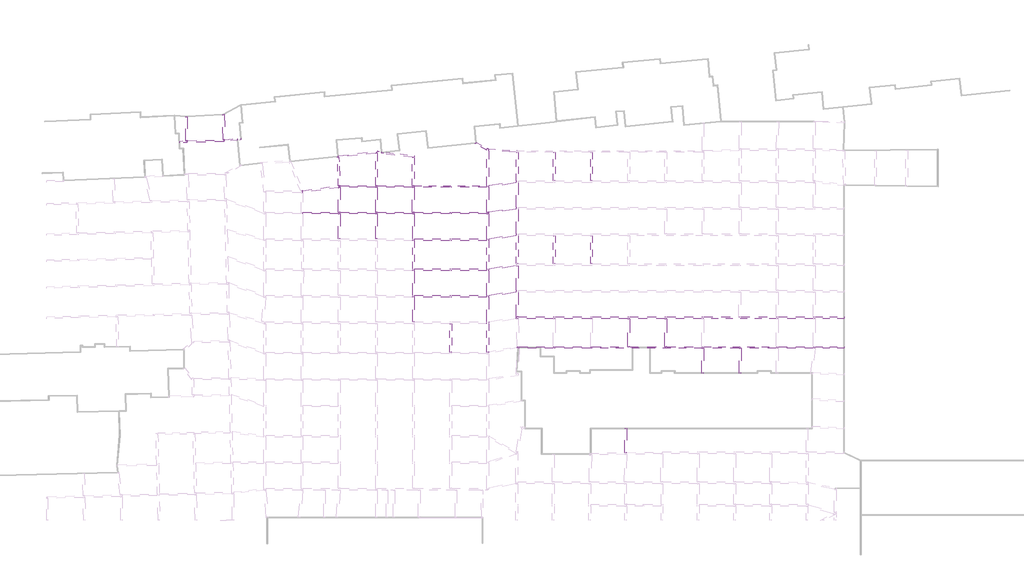
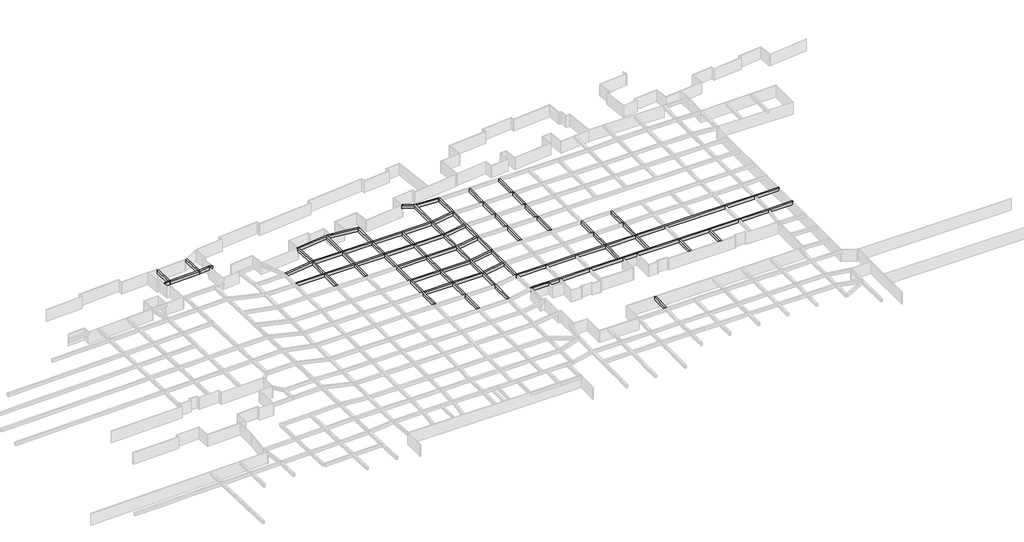
# One storey, part 19 of 20: 47 beams.
"""IFC4 building model written with IfcOpenShell, lengths in millimetres."""

from ifc_helpers import new_model, si_unit, frame, origin, place, context, project, spatial, polyline, outline, extrude, faceted_brep, element, save

model = new_model("IFC4")

# Units and contexts
model_context = context("Model", 3, world=origin())
ifc_project = project(units=[si_unit("LENGTHUNIT", "METRE", prefix="MILLI")], contexts=[model_context])

# Site, building, storey
site = spatial("IfcSite", under=ifc_project)
building = spatial("IfcBuilding", under=site)
storey = spatial("IfcBuildingStorey", under=building, Name="户型图", Elevation=0.0)

# Beams
placement = place(None, origin())
element("IfcBeam", 1, ObjectType="混凝土 - 矩形梁 : KL_beam", at=placement, inside=storey, context=model_context, shape_type="Brep", body=[
    faceted_brep([(37889.2589786, 194514.8382206, 3300.0), (37874.207263, 194914.598332, 3300.0), (37644.5215781, 194902.5610153, 3300.0), (36273.4586739, 194830.7066533, 3300.0), (36294.3930564, 194431.2548394, 3300.0), (37889.2589786, 194514.8382206, 2500.0), (36294.3930564, 194431.2548394, 2500.0), (37874.207263, 194914.598332, 2500.0), (36273.4586739, 194830.7066533, 2500.0), (37644.5215781, 194902.5610153, 2500.0)], [[[0, 1, 2, 3, 4]], [[5, 0, 4, 6]], [[7, 5, 6, 8, 9]], [[1, 7, 9, 8, 3, 2]], [[4, 3, 8, 6]], [[1, 0, 5, 7]]]),
])
element("IfcBeam", 2, ObjectType="混凝土 - 矩形梁 : KL_beam", at=placement, inside=storey, context=model_context, shape_type="Brep", body=[
    faceted_brep([(45868.2351761, 195097.7600189, 3300.0), (45638.7989465, 195092.5031037, 3300.0), (38044.2614823, 194918.4946679, 3300.0), (37874.207263, 194914.598332, 3300.0), (37889.2589786, 194514.8382206, 3300.0), (45893.7648239, 194698.2399811, 3300.0), (37889.2589786, 194514.8382206, 2500.0), (45893.7648239, 194698.2399811, 2500.0), (37874.207263, 194914.598332, 2500.0), (38044.2614823, 194918.4946679, 2500.0), (45638.7989465, 195092.5031037, 2500.0), (45868.2351761, 195097.7600189, 2500.0)], [[[0, 1, 2, 3, 4, 5]], [[5, 4, 6, 7]], [[7, 6, 8, 9, 10, 11]], [[3, 2, 1, 0, 11, 10, 9, 8]], [[3, 8, 6, 4]], [[0, 5, 7, 11]]]),
])
element("IfcBeam", 3, ObjectType="混凝土 - 矩形梁 : KL_beam", at=placement, inside=storey, context=model_context, shape_type="Brep", body=[
    faceted_brep([(45868.2351761, 195097.7600189, 3300.0), (45893.7648239, 194698.2399811, 3300.0), (48684.0697224, 194991.5128437, 3300.0), (48667.2783502, 195165.2272583, 3300.0), (48786.7216498, 195176.7727417, 3300.0), (48803.4165187, 195004.0566974, 3300.0), (49600.2651229, 195087.8088606, 3300.0), (49582.7742245, 195254.2236424, 3300.0), (49463.4315971, 195241.6802268, 3300.0), (49439.1111102, 195473.0742031, 3300.0), (46038.3737549, 195115.6423041, 3300.0), (49600.2651229, 195087.8088606, 2500.0), (48803.4165187, 195004.0566974, 2500.0), (45893.7648239, 194698.2399811, 2500.0), (45868.2351761, 195097.7600189, 2500.0), (46038.3737549, 195115.6423041, 2500.0), (49439.1111102, 195473.0742031, 2500.0), (49463.4315971, 195241.6802268, 2500.0), (49582.7742245, 195254.2236424, 2500.0), (48786.7216498, 195176.7727417, 2500.0), (48667.2783502, 195165.2272583, 2500.0), (48684.0697224, 194991.5128437, 2500.0)], [[[0, 1, 2, 3, 4, 5, 6, 7, 8, 9, 10]], [[11, 6, 5, 12]], [[13, 14, 15, 16, 17, 18, 11, 12, 19, 20, 21]], [[14, 0, 10, 9, 16, 15]], [[6, 11, 18, 7]], [[0, 14, 13, 1]], [[8, 17, 16, 9]], [[17, 8, 7, 18]], [[20, 3, 2, 21]], [[4, 19, 12, 5]], [[3, 20, 19, 4]], [[1, 13, 21, 2]]]),
])
element("IfcBeam", 4, ObjectType="混凝土 - 矩形梁 : KL_beam", at=placement, inside=storey, context=model_context, shape_type="SweptSolid", body=[
    extrude(outline(polyline([(37724.3604177, 200089.1615243), (37925.547951, 200099.7053161), (38044.2614823, 194918.4946679), (37874.207263, 194914.598332), (37644.5215781, 194902.5610153), (37525.4456991, 200099.586203), (37724.3604177, 200089.1615243)])), frame((0.0, 0.0, 2500.0), z_axis=(0.0, 0.0, 1.0), x_axis=(1.0, 0.0, 0.0)), (0.0, 0.0, 1.0), 800.0),
])
element("IfcBeam", 5, ObjectType="混凝土 - 矩形梁 : KL_beam", at=placement, inside=storey, context=model_context, shape_type="SweptSolid", body=[
    extrude(outline(polyline([(45729.8203033, 200508.709899), (45912.5795901, 200605.8847355), (46038.3737549, 195115.6423041), (45868.2351761, 195097.7600189), (45638.7989465, 195092.5031037), (45514.9591113, 200497.4495011), (45729.8203033, 200508.709899)])), frame((0.0, 0.0, 2500.0), z_axis=(0.0, 0.0, 1.0), x_axis=(1.0, 0.0, 0.0)), (0.0, 0.0, 1.0), 800.0),
])
element("IfcBeam", 6, ObjectType="混凝土 - 矩形梁 : KL_beam", at=placement, inside=storey, context=model_context, shape_type="Brep", body=[
    faceted_brep([(86850.0, 179140.0, 3300.0), (86850.0, 179540.0, 3300.0), (86806.9296004, 179540.0, 3300.0), (86406.9296004, 179540.0, 3300.0), (78866.5603873, 179540.0, 3300.0), (78466.5603873, 179540.0, 3300.0), (70871.1713568, 179540.0, 3300.0), (70471.1713568, 179540.0, 3300.0), (62850.0, 179540.0, 3300.0), (62850.0, 179140.0, 3300.0), (70471.1713568, 179140.0, 3300.0), (70871.1713568, 179140.0, 3300.0), (78466.5603873, 179140.0, 3300.0), (78866.5603873, 179140.0, 3300.0), (86450.0, 179140.0, 3300.0), (86850.0, 179140.0, 2500.0), (62850.0, 179140.0, 2500.0), (70471.1713568, 179140.0, 2500.0), (70871.1713568, 179140.0, 2500.0), (78466.5603873, 179140.0, 2500.0), (78866.5603873, 179140.0, 2500.0), (86450.0, 179140.0, 2500.0), (86850.0, 179540.0, 2500.0), (62850.0, 179540.0, 2500.0), (70471.1713568, 179540.0, 2500.0), (70871.1713568, 179540.0, 2500.0), (78466.5603873, 179540.0, 2500.0), (78866.5603873, 179540.0, 2500.0), (86406.9296004, 179540.0, 2500.0), (86806.9296004, 179540.0, 2500.0)], [[[0, 1, 2, 3, 4, 5, 6, 7, 8, 9, 10, 11, 12, 13, 14]], [[15, 0, 14, 13, 12, 11, 10, 9, 16, 17, 18, 19, 20, 21]], [[22, 15, 21, 20, 19, 18, 17, 16, 23, 24, 25, 26, 27, 28, 29]], [[1, 22, 29, 28, 27, 26, 25, 24, 23, 8, 7, 6, 5, 4, 3, 2]], [[9, 8, 23, 16]], [[1, 0, 15, 22]]]),
])
element("IfcBeam", 7, ObjectType="混凝土 - 矩形梁 : KL_beam", at=placement, inside=storey, context=model_context, shape_type="Brep", body=[
    faceted_brep([(70657.1859944, 185242.3021178, 3300.0), (70464.4923556, 185215.2207929, 3300.0), (62777.6028574, 184134.8989266, 3300.0), (62636.0146376, 184115.0, 3300.0), (62850.0, 184115.0, 3300.0), (62850.0, 183741.1426524, 3300.0), (70471.1713568, 184812.2284363, 3300.0), (70685.1567192, 184842.3021178, 3300.0), (62850.0, 183741.1426524, 2500.0), (70471.1713568, 184812.2284363, 2500.0), (70685.1567192, 184842.3021178, 2500.0), (62850.0, 184115.0, 2500.0), (62636.0146376, 184115.0, 2500.0), (62777.6028574, 184134.8989266, 2500.0), (70464.4923556, 185215.2207929, 2500.0), (70657.1859944, 185242.3021178, 2500.0)], [[[0, 1, 2, 3, 4, 5, 6, 7]], [[7, 6, 5, 8, 9, 10]], [[10, 9, 8, 11, 12, 13, 14, 15]], [[3, 2, 1, 0, 15, 14, 13, 12]], [[11, 4, 3, 12]], [[4, 11, 8, 5]], [[0, 7, 10, 15]]]),
])
element("IfcBeam", 8, ObjectType="混凝土 - 矩形梁 : KL_beam", at=placement, inside=storey, context=model_context, shape_type="Brep", body=[
    faceted_brep([(70657.1859944, 185242.3021178, 3300.0), (70685.1567192, 184842.3021178, 3300.0), (70871.1713568, 184842.3021178, 3300.0), (78466.5603873, 184842.3021178, 3300.0), (78866.5603873, 184842.3021178, 3300.0), (86406.9296004, 184842.3021178, 3300.0), (86806.9296004, 184842.3021178, 3300.0), (86806.9296004, 185242.3021178, 3300.0), (86406.9296004, 185242.3021178, 3300.0), (78866.5603873, 185242.3021178, 3300.0), (78466.5603873, 185242.3021178, 3300.0), (70863.7543579, 185242.3021178, 3300.0), (70685.1567192, 184842.3021178, 2500.0), (70871.1713568, 184842.3021178, 2500.0), (78466.5603873, 184842.3021178, 2500.0), (78866.5603873, 184842.3021178, 2500.0), (86406.9296004, 184842.3021178, 2500.0), (86806.9296004, 184842.3021178, 2500.0), (70657.1859944, 185242.3021178, 2500.0), (70863.7543579, 185242.3021178, 2500.0), (78466.5603873, 185242.3021178, 2500.0), (78866.5603873, 185242.3021178, 2500.0), (86406.9296004, 185242.3021178, 2500.0), (86806.9296004, 185242.3021178, 2500.0)], [[[0, 1, 2, 3, 4, 5, 6, 7, 8, 9, 10, 11]], [[1, 12, 13, 14, 15, 16, 17, 6, 5, 4, 3, 2]], [[12, 18, 19, 20, 21, 22, 23, 17, 16, 15, 14, 13]], [[18, 0, 11, 10, 9, 8, 7, 23, 22, 21, 20, 19]], [[0, 18, 12, 1]], [[7, 6, 17, 23]]]),
])
element("IfcBeam", 9, ObjectType="混凝土 - 矩形梁 : KL_beam", at=placement, inside=storey, context=model_context, shape_type="Brep", body=[
    faceted_brep([(70707.0899583, 189386.9587472, 3300.0), (70508.8980465, 191272.6288285, 3300.0), (70494.4229915, 191410.349777, 3300.0), (70231.283324, 191384.9144894, 3300.0), (70464.4923556, 185215.2207929, 3300.0), (70657.1859944, 185242.3021178, 3300.0), (70863.7543579, 185242.3021178, 3300.0), (70464.4923556, 185215.2207929, 2500.0), (70231.283324, 191384.9144894, 2500.0), (70494.4229915, 191410.349777, 2500.0), (70508.8980465, 191272.6288285, 2500.0), (70707.0899583, 189386.9587472, 2500.0), (70863.7543579, 185242.3021178, 2500.0), (70657.1859944, 185242.3021178, 2500.0)], [[[0, 1, 2, 3, 4, 5, 6]], [[7, 4, 3, 8]], [[8, 9, 10, 11, 12, 13, 7]], [[11, 0, 6, 12]], [[0, 11, 10, 9, 2, 1]], [[2, 9, 8, 3]], [[5, 4, 7, 13]], [[6, 5, 13, 12]]]),
])
element("IfcBeam", 10, ObjectType="混凝土 - 矩形梁 : KL_beam", at=placement, inside=storey, context=model_context, shape_type="Brep", body=[
    faceted_brep([(78817.8126499, 192695.8391898, 3300.0), (70467.0802921, 191670.498184, 3300.0), (70494.4229915, 191410.349777, 3300.0), (70508.8980465, 191272.6288285, 3300.0), (78466.5603873, 192249.7069048, 3300.0), (78866.5603873, 192298.8207291, 3300.0), (78822.4430306, 192658.1277652, 3300.0), (70508.8980465, 191272.6288285, 2500.0), (78466.5603873, 192249.7069048, 2500.0), (78866.5603873, 192298.8207291, 2500.0), (70467.0802921, 191670.498184, 2500.0), (78817.8126499, 192695.8391898, 2500.0), (78822.4430306, 192658.1277652, 2500.0), (70494.4229915, 191410.349777, 2500.0)], [[[0, 1, 2, 3, 4, 5, 6]], [[5, 4, 3, 7, 8, 9]], [[10, 11, 12, 9, 8, 7, 13]], [[1, 0, 11, 10]], [[1, 10, 13, 7, 3, 2]], [[0, 6, 5, 9, 12, 11]]]),
    faceted_brep([(70221.627692, 191640.3603943, 3300.0), (70221.627692, 191640.3603943, 2500.0), (70226.7428774, 191505.0349014, 2500.0), (70226.7428774, 191505.0349014, 3300.0), (70347.9566108, 191655.8716351, 2500.0), (70347.9566108, 191655.8716351, 3300.0), (70362.4316658, 191518.1506866, 3300.0), (70362.4316658, 191518.1506866, 2500.0)], [[[0, 1, 2, 3]], [[4, 5, 6, 7]], [[1, 0, 5, 4]], [[6, 3, 2, 7]], [[5, 0, 3, 6]], [[1, 4, 7, 2]]]),
])
element("IfcBeam", 11, ObjectType="混凝土 - 矩形梁 : KL_beam", at=placement, inside=storey, context=model_context, shape_type="Brep", body=[
    faceted_brep([(78866.5603873, 192298.8207291, 3300.0), (78466.5603873, 192249.7069048, 3300.0), (78466.5603873, 185242.3021178, 3300.0), (78866.5603873, 185242.3021178, 3300.0), (78866.5603873, 192249.7069048, 3300.0), (78466.5603873, 192249.7069048, 2500.0), (78466.5603873, 185242.3021178, 2500.0), (78866.5603873, 192298.8207291, 2500.0), (78866.5603873, 192249.7069048, 2500.0), (78866.5603873, 185242.3021178, 2500.0)], [[[0, 1, 2, 3, 4]], [[1, 5, 6, 2]], [[5, 7, 8, 9, 6]], [[7, 0, 4, 3, 9, 8]], [[1, 0, 7, 5]], [[3, 2, 6, 9]]]),
])
element("IfcBeam", 12, ObjectType="混凝土 - 矩形梁 : KL_beam", at=placement, inside=storey, context=model_context, shape_type="Brep", body=[
    faceted_brep([(79847.9790856, 192432.6191009, 3300.0), (80284.9846417, 192478.5502357, 3300.0), (79837.3750476, 192533.5097832, 3300.0), (80284.9846417, 192478.5502357, 2500.0), (79847.9790856, 192432.6191009, 2500.0), (79837.3750476, 192533.5097832, 2500.0)], [[[0, 1, 2]], [[3, 4, 5]], [[3, 1, 0, 4]], [[1, 3, 5, 2]], [[0, 2, 5, 4]]]),
    faceted_brep([(78866.5603873, 192249.7069048, 3300.0), (78866.5603873, 192249.7069048, 2500.0), (86406.9296004, 191323.8659819, 2500.0), (86806.9296004, 191274.7521575, 2500.0), (86806.9296004, 191274.7521575, 3300.0), (86406.9296004, 191323.8659819, 3300.0), (80814.4577688, 192413.5391103, 2500.0), (80814.4577688, 192413.5391103, 3300.0), (86806.9296004, 191677.7560877, 3300.0), (86806.9296004, 191677.7560877, 2500.0), (78866.5603873, 192298.8207291, 3300.0), (78822.4430306, 192658.1277652, 3300.0), (78822.4430306, 192658.1277652, 2500.0), (78866.5603873, 192298.8207291, 2500.0), (79741.1798737, 192300.7330579, 2500.0), (79741.1798737, 192300.7330579, 3300.0), (79715.1365445, 192548.5187841, 2500.0), (79715.1365445, 192548.5187841, 3300.0), (79728.6364581, 192420.0756853, 3300.0)], [[[0, 1, 2, 3, 4, 5]], [[6, 7, 8, 9]], [[10, 11, 12, 13]], [[0, 10, 13, 1]], [[14, 15, 7, 6]], [[15, 14, 16, 17, 18]], [[11, 10, 0, 5, 4, 8, 7, 15, 18, 17]], [[13, 12, 16, 14, 6, 9, 3, 2, 1]], [[12, 11, 17, 16]], [[8, 4, 3, 9]]]),
])
element("IfcBeam", 13, ObjectType="混凝土 - 矩形梁 : KL_beam", at=placement, inside=storey, context=model_context, shape_type="SweptSolid", body=[
    extrude(outline(polyline([(86806.9296004, 185242.3021178), (86406.9296004, 185242.3021178), (86406.9296004, 191323.8659819), (86806.9296004, 191274.7521575), (86806.9296004, 185242.3021178)])), frame((0.0, 0.0, 2500.0), z_axis=(0.0, 0.0, 1.0), x_axis=(1.0, 0.0, 0.0)), (0.0, 0.0, 1.0), 800.0),
])
element("IfcBeam", 14, ObjectType="混凝土 - 矩形梁 : KL_beam", at=placement, inside=storey, context=model_context, shape_type="Brep", body=[
    faceted_brep([(70871.1713568, 184842.3021178, 3300.0), (70685.1567192, 184842.3021178, 3300.0), (70479.6799144, 184813.4242361, 3300.0), (70471.1713568, 184812.2284363, 3300.0), (70471.1713568, 179540.0, 3300.0), (70871.1713568, 179540.0, 3300.0), (70471.1713568, 184812.2284363, 2500.0), (70471.1713568, 179540.0, 2500.0), (70685.1567192, 184842.3021178, 2500.0), (70871.1713568, 184842.3021178, 2500.0), (70871.1713568, 179540.0, 2500.0), (70479.6799144, 184813.4242361, 2500.0)], [[[0, 1, 2, 3, 4, 5]], [[3, 6, 7, 4]], [[8, 9, 10, 7, 6, 11]], [[9, 0, 5, 10]], [[6, 3, 2, 1, 8, 11]], [[1, 0, 9, 8]], [[5, 4, 7, 10]]]),
])
element("IfcBeam", 15, ObjectType="混凝土 - 矩形梁 : KL_beam", at=placement, inside=storey, context=model_context, shape_type="SweptSolid", body=[
    extrude(outline(polyline([(70871.1713568, 173790.0), (70471.1713568, 173790.0), (70471.1713568, 179140.0), (70871.1713568, 179140.0), (70871.1713568, 173790.0)])), frame((0.0, 0.0, 2500.0), z_axis=(0.0, 0.0, 1.0), x_axis=(1.0, 0.0, 0.0)), (0.0, 0.0, 1.0), 800.0),
])
element("IfcBeam", 16, ObjectType="混凝土 - 矩形梁 : KL_beam", at=placement, inside=storey, context=model_context, shape_type="SweptSolid", body=[
    extrude(outline(polyline([(78866.5603873, 179540.0), (78466.5603873, 179540.0), (78466.5603873, 184842.3021178), (78866.5603873, 184842.3021178), (78866.5603873, 179540.0)])), frame((0.0, 0.0, 2500.0), z_axis=(0.0, 0.0, 1.0), x_axis=(1.0, 0.0, 0.0)), (0.0, 0.0, 1.0), 800.0),
])
element("IfcBeam", 17, ObjectType="混凝土 - 矩形梁 : KL_beam", at=placement, inside=storey, context=model_context, shape_type="SweptSolid", body=[
    extrude(outline(polyline([(78866.5603873, 173790.0), (78466.5603873, 173790.0), (78466.5603873, 179140.0), (78866.5603873, 179140.0), (78866.5603873, 173790.0)])), frame((0.0, 0.0, 2500.0), z_axis=(0.0, 0.0, 1.0), x_axis=(1.0, 0.0, 0.0)), (0.0, 0.0, 1.0), 800.0),
])
element("IfcBeam", 18, ObjectType="混凝土 - 矩形梁 : KL_beam", at=placement, inside=storey, context=model_context, shape_type="Brep", body=[
    faceted_brep([(86450.0, 155890.0, 3300.0), (86850.0, 155890.0, 3300.0), (86850.0, 161190.0, 3300.0), (86850.0, 161590.0, 3300.0), (86850.0, 166890.0, 3300.0), (86850.0, 167290.0, 3300.0), (86850.0, 173390.0, 3300.0), (86850.0, 173790.0, 3300.0), (86850.0, 179140.0, 3300.0), (86450.0, 179140.0, 3300.0), (86450.0, 173790.0, 3300.0), (86450.0, 173390.0, 3300.0), (86450.0, 167290.0, 3300.0), (86450.0, 166890.0, 3300.0), (86450.0, 161590.0, 3300.0), (86450.0, 161190.0, 3300.0), (86450.0, 155890.0, 2500.0), (86450.0, 179140.0, 2500.0), (86450.0, 173790.0, 2500.0), (86450.0, 173390.0, 2500.0), (86450.0, 167290.0, 2500.0), (86450.0, 166890.0, 2500.0), (86450.0, 161590.0, 2500.0), (86450.0, 161190.0, 2500.0), (86850.0, 155890.0, 2500.0), (86850.0, 179140.0, 2500.0), (86850.0, 173790.0, 2500.0), (86850.0, 173390.0, 2500.0), (86850.0, 167290.0, 2500.0), (86850.0, 166890.0, 2500.0), (86850.0, 161590.0, 2500.0), (86850.0, 161190.0, 2500.0)], [[[0, 1, 2, 3, 4, 5, 6, 7, 8, 9, 10, 11, 12, 13, 14, 15]], [[16, 0, 15, 14, 13, 12, 11, 10, 9, 17, 18, 19, 20, 21, 22, 23]], [[24, 16, 23, 22, 21, 20, 19, 18, 17, 25, 26, 27, 28, 29, 30, 31]], [[1, 24, 31, 30, 29, 28, 27, 26, 25, 8, 7, 6, 5, 4, 3, 2]], [[1, 0, 16, 24]], [[9, 8, 25, 17]]]),
])
element("IfcBeam", 19, ObjectType="混凝土 - 矩形梁 : KL_beam", at=placement, inside=storey, context=model_context, shape_type="Brep", body=[
    faceted_brep([(86850.0, 161590.0, 3300.0), (86850.0, 161190.0, 3300.0), (94423.4648002, 161190.0, 3300.0), (94823.4648002, 161190.0, 3300.0), (102450.0, 161190.0, 3300.0), (102450.0, 161590.0, 3300.0), (94823.4648002, 161590.0, 3300.0), (94423.4648002, 161590.0, 3300.0), (86850.0, 161190.0, 2500.0), (94423.4648002, 161190.0, 2500.0), (94823.4648002, 161190.0, 2500.0), (102450.0, 161190.0, 2500.0), (86850.0, 161590.0, 2500.0), (94423.4648002, 161590.0, 2500.0), (94823.4648002, 161590.0, 2500.0), (102450.0, 161590.0, 2500.0)], [[[0, 1, 2, 3, 4, 5, 6, 7]], [[1, 8, 9, 10, 11, 4, 3, 2]], [[8, 12, 13, 14, 15, 11, 10, 9]], [[12, 0, 7, 6, 5, 15, 14, 13]], [[1, 0, 12, 8]], [[5, 4, 11, 15]]]),
])
element("IfcBeam", 20, ObjectType="混凝土 - 矩形梁 : KL_beam", at=placement, inside=storey, context=model_context, shape_type="Brep", body=[
    faceted_brep([(86850.0, 167290.0, 3300.0), (86850.0, 166890.0, 3300.0), (94423.4648002, 166890.0, 3300.0), (94823.4648002, 166890.0, 3300.0), (102450.0, 166890.0, 3300.0), (102450.0, 167290.0, 3300.0), (94823.4648002, 167290.0, 3300.0), (94423.4648002, 167290.0, 3300.0), (86850.0, 166890.0, 2500.0), (94423.4648002, 166890.0, 2500.0), (94823.4648002, 166890.0, 2500.0), (102450.0, 166890.0, 2500.0), (86850.0, 167290.0, 2500.0), (94423.4648002, 167290.0, 2500.0), (94823.4648002, 167290.0, 2500.0), (102450.0, 167290.0, 2500.0)], [[[0, 1, 2, 3, 4, 5, 6, 7]], [[1, 8, 9, 10, 11, 4, 3, 2]], [[8, 12, 13, 14, 15, 11, 10, 9]], [[12, 0, 7, 6, 5, 15, 14, 13]], [[1, 0, 12, 8]], [[5, 4, 11, 15]]]),
])
element("IfcBeam", 21, ObjectType="混凝土 - 矩形梁 : KL_beam", at=placement, inside=storey, context=model_context, shape_type="Brep", body=[
    faceted_brep([(86850.0, 173790.0, 3300.0), (86850.0, 173390.0, 3300.0), (94423.4648002, 173390.0, 3300.0), (94823.4648002, 173390.0, 3300.0), (102450.0, 173390.0, 3300.0), (102450.0, 173790.0, 3300.0), (94823.4648002, 173790.0, 3300.0), (94423.4648002, 173790.0, 3300.0), (86850.0, 173390.0, 2500.0), (94423.4648002, 173390.0, 2500.0), (94823.4648002, 173390.0, 2500.0), (102450.0, 173390.0, 2500.0), (86850.0, 173790.0, 2500.0), (94423.4648002, 173790.0, 2500.0), (94823.4648002, 173790.0, 2500.0), (102450.0, 173790.0, 2500.0)], [[[0, 1, 2, 3, 4, 5, 6, 7]], [[1, 8, 9, 10, 11, 4, 3, 2]], [[8, 12, 13, 14, 15, 11, 10, 9]], [[12, 0, 7, 6, 5, 15, 14, 13]], [[1, 0, 12, 8]], [[5, 4, 11, 15]]]),
])
element("IfcBeam", 22, ObjectType="混凝土 - 矩形梁 : KL_beam", at=placement, inside=storey, context=model_context, shape_type="Brep", body=[
    faceted_brep([(102850.0, 179140.0, 3300.0), (102850.0, 179170.5745823, 3300.0), (102850.0, 179540.0, 3300.0), (102450.0, 179540.0, 3300.0), (94823.4648002, 179540.0, 3300.0), (94423.4648002, 179540.0, 3300.0), (86850.0, 179540.0, 3300.0), (86850.0, 179140.0, 3300.0), (94423.4648002, 179140.0, 3300.0), (94823.4648002, 179140.0, 3300.0), (102450.0, 179140.0, 3300.0), (102850.0, 179140.0, 2500.0), (86850.0, 179140.0, 2500.0), (94423.4648002, 179140.0, 2500.0), (94823.4648002, 179140.0, 2500.0), (102450.0, 179140.0, 2500.0), (102850.0, 179540.0, 2500.0), (102850.0, 179170.5745823, 2500.0), (86850.0, 179540.0, 2500.0), (94423.4648002, 179540.0, 2500.0), (94823.4648002, 179540.0, 2500.0), (102450.0, 179540.0, 2500.0)], [[[0, 1, 2, 3, 4, 5, 6, 7, 8, 9, 10]], [[11, 0, 10, 9, 8, 7, 12, 13, 14, 15]], [[16, 17, 11, 15, 14, 13, 12, 18, 19, 20, 21]], [[2, 16, 21, 20, 19, 18, 6, 5, 4, 3]], [[7, 6, 18, 12]], [[2, 1, 0, 11, 17, 16]]]),
])
element("IfcBeam", 23, ObjectType="混凝土 - 矩形梁 : KL_beam", at=placement, inside=storey, context=model_context, shape_type="SweptSolid", body=[
    extrude(outline(polyline([(86806.9296004, 179540.0), (86406.9296004, 179540.0), (86406.9296004, 184842.3021178), (86806.9296004, 184842.3021178), (86806.9296004, 179540.0)])), frame((0.0, 0.0, 2500.0), z_axis=(0.0, 0.0, 1.0), x_axis=(1.0, 0.0, 0.0)), (0.0, 0.0, 1.0), 800.0),
])
element("IfcBeam", 24, ObjectType="混凝土 - 矩形梁 : KL_beam", at=placement, inside=storey, context=model_context, shape_type="Brep", body=[
    faceted_brep([(86806.9296004, 185242.3021178, 3300.0), (86806.9296004, 184842.3021178, 3300.0), (94423.4648002, 184842.3021178, 3300.0), (94823.4648002, 184842.3021178, 3300.0), (102450.0, 184842.3021178, 3300.0), (102450.0, 185242.3021178, 3300.0), (86806.9296004, 184842.3021178, 2500.0), (94423.4648002, 184842.3021178, 2500.0), (94823.4648002, 184842.3021178, 2500.0), (102450.0, 184842.3021178, 2500.0), (86806.9296004, 185242.3021178, 2500.0), (102450.0, 185242.3021178, 2500.0)], [[[0, 1, 2, 3, 4, 5]], [[1, 6, 7, 8, 9, 4, 3, 2]], [[6, 10, 11, 9, 8, 7]], [[10, 0, 5, 11]], [[1, 0, 10, 6]], [[5, 4, 9, 11]]]),
])
element("IfcBeam", 25, ObjectType="混凝土 - 矩形梁 : KL_beam", at=placement, inside=storey, context=model_context, shape_type="SweptSolid", body=[
    extrude(outline(polyline([(94423.4648002, 184842.3021178), (94823.4648002, 184842.3021178), (94823.4648002, 179540.0), (94423.4648002, 179540.0), (94423.4648002, 184842.3021178)])), frame((0.0, 0.0, 2500.0), z_axis=(0.0, 0.0, 1.0), x_axis=(1.0, 0.0, 0.0)), (0.0, 0.0, 1.0), 800.0),
    extrude(outline(polyline([(94423.4648002, 155490.0), (94823.4648002, 155490.0), (94823.4648002, 149390.0), (94423.4648002, 149390.0), (94423.4648002, 155490.0)])), frame((0.0, 0.0, 2500.0), z_axis=(0.0, 0.0, 1.0), x_axis=(1.0, 0.0, 0.0)), (0.0, 0.0, 1.0), 800.0),
    extrude(outline(polyline([(94823.4648002, 155890.0), (94423.4648002, 155890.0), (94423.4648002, 161190.0), (94823.4648002, 161190.0), (94823.4648002, 155890.0)])), frame((0.0, 0.0, 2500.0), z_axis=(0.0, 0.0, 1.0), x_axis=(1.0, 0.0, 0.0)), (0.0, 0.0, 1.0), 800.0),
    extrude(outline(polyline([(94823.4648002, 161590.0), (94423.4648002, 161590.0), (94423.4648002, 166890.0), (94823.4648002, 166890.0), (94823.4648002, 161590.0)])), frame((0.0, 0.0, 2500.0), z_axis=(0.0, 0.0, 1.0), x_axis=(1.0, 0.0, 0.0)), (0.0, 0.0, 1.0), 800.0),
    extrude(outline(polyline([(94823.4648002, 167290.0), (94423.4648002, 167290.0), (94423.4648002, 173390.0), (94823.4648002, 173390.0), (94823.4648002, 167290.0)])), frame((0.0, 0.0, 2500.0), z_axis=(0.0, 0.0, 1.0), x_axis=(1.0, 0.0, 0.0)), (0.0, 0.0, 1.0), 800.0),
    extrude(outline(polyline([(94823.4648002, 173790.0), (94423.4648002, 173790.0), (94423.4648002, 179140.0), (94823.4648002, 179140.0), (94823.4648002, 173790.0)])), frame((0.0, 0.0, 2500.0), z_axis=(0.0, 0.0, 1.0), x_axis=(1.0, 0.0, 0.0)), (0.0, 0.0, 1.0), 800.0),
])
element("IfcBeam", 26, ObjectType="混凝土 - 矩形梁 : KL_beam", at=placement, inside=storey, context=model_context, shape_type="Brep", body=[
    faceted_brep([(102850.0, 179140.0, 3300.0), (102450.0, 179140.0, 3300.0), (102450.0, 173790.0, 3300.0), (102450.0, 173390.0, 3300.0), (102450.0, 167290.0, 3300.0), (102450.0, 166890.0, 3300.0), (102450.0, 161590.0, 3300.0), (102450.0, 161190.0, 3300.0), (102450.0, 155890.0, 3300.0), (102450.0, 155490.0, 3300.0), (102450.0, 149390.0, 3300.0), (102850.0, 149390.0, 3300.0), (102850.0, 149435.3885337, 3300.0), (102850.0, 155521.8686077, 3300.0), (102850.0, 155927.9091701, 3300.0), (102850.0, 161221.8686077, 3300.0), (102850.0, 161627.9091701, 3300.0), (102850.0, 166921.8686077, 3300.0), (102850.0, 167327.9091701, 3300.0), (102850.0, 173421.8686077, 3300.0), (102850.0, 173827.9091701, 3300.0), (102450.0, 179140.0, 2500.0), (102450.0, 173790.0, 2500.0), (102450.0, 173390.0, 2500.0), (102450.0, 167290.0, 2500.0), (102450.0, 166890.0, 2500.0), (102450.0, 161590.0, 2500.0), (102450.0, 161190.0, 2500.0), (102450.0, 155890.0, 2500.0), (102450.0, 155490.0, 2500.0), (102450.0, 149390.0, 2500.0), (102850.0, 179140.0, 2500.0), (102850.0, 173827.9091701, 2500.0), (102850.0, 173421.8686077, 2500.0), (102850.0, 167327.9091701, 2500.0), (102850.0, 166921.8686077, 2500.0), (102850.0, 161627.9091701, 2500.0), (102850.0, 161221.8686077, 2500.0), (102850.0, 155927.9091701, 2500.0), (102850.0, 155521.8686077, 2500.0), (102850.0, 149435.3885337, 2500.0), (102850.0, 149390.0, 2500.0)], [[[0, 1, 2, 3, 4, 5, 6, 7, 8, 9, 10, 11, 12, 13, 14, 15, 16, 17, 18, 19, 20]], [[1, 21, 22, 23, 24, 25, 26, 27, 28, 29, 30, 10, 9, 8, 7, 6, 5, 4, 3, 2]], [[21, 31, 32, 33, 34, 35, 36, 37, 38, 39, 40, 41, 30, 29, 28, 27, 26, 25, 24, 23, 22]], [[31, 0, 20, 19, 18, 17, 16, 15, 14, 13, 12, 11, 41, 40, 39, 38, 37, 36, 35, 34, 33, 32]], [[1, 0, 31, 21]], [[11, 10, 30, 41]]]),
])
element("IfcBeam", 27, ObjectType="混凝土 - 矩形梁 : KL_beam", at=placement, inside=storey, context=model_context, shape_type="Brep", body=[
    faceted_brep([(179400.0, 156989.0, 3300.0), (179400.0, 156589.0, 3300.0), (179400.0, 156589.0, 2500.0), (179400.0, 156989.0, 2500.0), (173150.0, 156989.0, 3300.0), (172750.0, 156989.0, 3300.0), (165150.0, 156989.0, 3300.0), (164750.0, 156989.0, 3300.0), (157079.0, 156989.0, 3300.0), (156679.0, 156989.0, 3300.0), (149149.0, 156989.0, 3300.0), (148749.0, 156989.0, 3300.0), (141149.0, 156989.0, 3300.0), (140749.0, 156989.0, 3300.0), (133150.0, 156989.0, 3300.0), (132750.0, 156989.0, 3300.0), (125150.0, 156989.0, 3300.0), (124750.0, 156989.0, 3300.0), (117150.0, 156989.0, 3300.0), (116750.0, 156989.0, 3300.0), (109150.0, 156989.0, 3300.0), (108750.0, 156989.0, 3300.0), (108750.0, 156957.1313923, 3300.0), (108750.0, 156785.0903557, 3300.0), (108750.0, 156589.0, 3300.0), (108757.6693662, 156589.0, 3300.0), (109157.9751895, 156589.0, 3300.0), (116750.0, 156589.0, 3300.0), (117150.0, 156589.0, 3300.0), (124750.0, 156589.0, 3300.0), (125150.0, 156589.0, 3300.0), (132750.0, 156589.0, 3300.0), (133150.0, 156589.0, 3300.0), (140749.0, 156589.0, 3300.0), (141149.0, 156589.0, 3300.0), (148749.0, 156589.0, 3300.0), (149149.0, 156589.0, 3300.0), (164750.0, 156589.0, 3300.0), (165150.0, 156589.0, 3300.0), (172750.0, 156589.0, 3300.0), (173150.0, 156589.0, 3300.0), (108750.0, 156589.0, 2500.0), (108757.6693662, 156589.0, 2500.0), (109157.9751895, 156589.0, 2500.0), (116750.0, 156589.0, 2500.0), (117150.0, 156589.0, 2500.0), (124750.0, 156589.0, 2500.0), (125150.0, 156589.0, 2500.0), (132750.0, 156589.0, 2500.0), (133150.0, 156589.0, 2500.0), (140749.0, 156589.0, 2500.0), (141149.0, 156589.0, 2500.0), (148749.0, 156589.0, 2500.0), (149149.0, 156589.0, 2500.0), (164750.0, 156589.0, 2500.0), (165150.0, 156589.0, 2500.0), (172750.0, 156589.0, 2500.0), (173150.0, 156589.0, 2500.0), (108750.0, 156785.0903557, 2500.0), (108750.0, 156957.1313923, 2500.0), (108750.0, 156989.0, 2500.0), (109150.0, 156989.0, 2500.0), (116750.0, 156989.0, 2500.0), (117150.0, 156989.0, 2500.0), (124750.0, 156989.0, 2500.0), (125150.0, 156989.0, 2500.0), (132750.0, 156989.0, 2500.0), (133150.0, 156989.0, 2500.0), (140749.0, 156989.0, 2500.0), (141149.0, 156989.0, 2500.0), (148749.0, 156989.0, 2500.0), (149149.0, 156989.0, 2500.0), (156679.0, 156989.0, 2500.0), (157079.0, 156989.0, 2500.0), (164750.0, 156989.0, 2500.0), (165150.0, 156989.0, 2500.0), (172750.0, 156989.0, 2500.0), (173150.0, 156989.0, 2500.0)], [[[0, 1, 2, 3]], [[1, 0, 4, 5, 6, 7, 8, 9, 10, 11, 12, 13, 14, 15, 16, 17, 18, 19, 20, 21, 22, 23, 24, 25, 26, 27, 28, 29, 30, 31, 32, 33, 34, 35, 36, 37, 38, 39, 40]], [[2, 1, 40, 39, 38, 37, 36, 35, 34, 33, 32, 31, 30, 29, 28, 27, 26, 25, 24, 41, 42, 43, 44, 45, 46, 47, 48, 49, 50, 51, 52, 53, 54, 55, 56, 57]], [[3, 2, 57, 56, 55, 54, 53, 52, 51, 50, 49, 48, 47, 46, 45, 44, 43, 42, 41, 58, 59, 60, 61, 62, 63, 64, 65, 66, 67, 68, 69, 70, 71, 72, 73, 74, 75, 76, 77]], [[0, 3, 77, 76, 75, 74, 73, 72, 71, 70, 69, 68, 67, 66, 65, 64, 63, 62, 61, 60, 21, 20, 19, 18, 17, 16, 15, 14, 13, 12, 11, 10, 9, 8, 7, 6, 5, 4]], [[24, 23, 22, 21, 60, 59, 58, 41]]]),
])
element("IfcBeam", 28, ObjectType="混凝土 - 矩形梁 : KL_beam", at=placement, inside=storey, context=model_context, shape_type="Brep", body=[
    faceted_brep([(179419.9999913, 150597.0, 3300.0), (179419.9999913, 150197.0, 3300.0), (179419.9999913, 150197.0, 2500.0), (179419.9999913, 150597.0, 2500.0), (173150.0, 150597.0, 3300.0), (172750.0, 150597.0, 3300.0), (165150.0, 150597.0, 3300.0), (164750.0, 150597.0, 3300.0), (149149.0, 150597.0, 3300.0), (148749.0, 150597.0, 3300.0), (141149.0, 150597.0, 3300.0), (140749.0, 150597.0, 3300.0), (133150.0, 150597.0, 3300.0), (132750.0, 150597.0, 3300.0), (125150.0, 150597.0, 3300.0), (124750.0, 150597.0, 3300.0), (117150.0, 150597.0, 3300.0), (116750.0, 150597.0, 3300.0), (109392.3306338, 150597.0, 3300.0), (108992.0248105, 150597.0, 3300.0), (109003.8596337, 150294.4072408, 3300.0), (109007.6693662, 150197.0, 3300.0), (109392.4019191, 150197.0, 3300.0), (116750.0, 150197.0, 3300.0), (117150.0, 150197.0, 3300.0), (124750.0, 150197.0, 3300.0), (125150.0, 150197.0, 3300.0), (148749.0, 150197.0, 3300.0), (149149.0, 150197.0, 3300.0), (156779.0, 150197.0, 3300.0), (157179.0, 150197.0, 3300.0), (164750.0, 150197.0, 3300.0), (165150.0, 150197.0, 3300.0), (172727.877497, 150197.0, 3300.0), (173130.0808089, 150197.0, 3300.0), (109007.6693662, 150197.0, 2500.0), (109392.4019191, 150197.0, 2500.0), (116750.0, 150197.0, 2500.0), (117150.0, 150197.0, 2500.0), (124750.0, 150197.0, 2500.0), (125150.0, 150197.0, 2500.0), (148749.0, 150197.0, 2500.0), (149149.0, 150197.0, 2500.0), (156779.0, 150197.0, 2500.0), (157179.0, 150197.0, 2500.0), (164750.0, 150197.0, 2500.0), (165150.0, 150197.0, 2500.0), (172727.877497, 150197.0, 2500.0), (173130.0808089, 150197.0, 2500.0), (109003.8596337, 150294.4072408, 2500.0), (108992.0248105, 150597.0, 2500.0), (109392.3306338, 150597.0, 2500.0), (116750.0, 150597.0, 2500.0), (117150.0, 150597.0, 2500.0), (124750.0, 150597.0, 2500.0), (125150.0, 150597.0, 2500.0), (132750.0, 150597.0, 2500.0), (133150.0, 150597.0, 2500.0), (140749.0, 150597.0, 2500.0), (141149.0, 150597.0, 2500.0), (148749.0, 150597.0, 2500.0), (149149.0, 150597.0, 2500.0), (164750.0, 150597.0, 2500.0), (165150.0, 150597.0, 2500.0), (172750.0, 150597.0, 2500.0), (173150.0, 150597.0, 2500.0)], [[[0, 1, 2, 3]], [[1, 0, 4, 5, 6, 7, 8, 9, 10, 11, 12, 13, 14, 15, 16, 17, 18, 19, 20, 21, 22, 23, 24, 25, 26, 27, 28, 29, 30, 31, 32, 33, 34]], [[2, 1, 34, 33, 32, 31, 30, 29, 28, 27, 26, 25, 24, 23, 22, 21, 35, 36, 37, 38, 39, 40, 41, 42, 43, 44, 45, 46, 47, 48]], [[3, 2, 48, 47, 46, 45, 44, 43, 42, 41, 40, 39, 38, 37, 36, 35, 49, 50, 51, 52, 53, 54, 55, 56, 57, 58, 59, 60, 61, 62, 63, 64, 65]], [[0, 3, 65, 64, 63, 62, 61, 60, 59, 58, 57, 56, 55, 54, 53, 52, 51, 50, 19, 18, 17, 16, 15, 14, 13, 12, 11, 10, 9, 8, 7, 6, 5, 4]], [[21, 20, 19, 50, 49, 35]]]),
])
element("IfcBeam", 29, ObjectType="混凝土 - 矩形梁 : KL_beam", at=placement, inside=storey, context=model_context, shape_type="SweptSolid", body=[
    extrude(outline(polyline([(124750.0, 192389.0), (125150.0, 192389.0), (125150.0, 186289.0), (124750.0, 186289.0), (124750.0, 192389.0)])), frame((0.0, 0.0, 2500.0), z_axis=(0.0, 0.0, 1.0), x_axis=(1.0, 0.0, 0.0)), (0.0, 0.0, 1.0), 800.0),
    extrude(outline(polyline([(125150.0, 180590.0), (124750.0, 180590.0), (124750.0, 185889.0), (125150.0, 185889.0), (125150.0, 180590.0)])), frame((0.0, 0.0, 2500.0), z_axis=(0.0, 0.0, 1.0), x_axis=(1.0, 0.0, 0.0)), (0.0, 0.0, 1.0), 800.0),
])
element("IfcBeam", 30, ObjectType="混凝土 - 矩形梁 : KL_beam", at=placement, inside=storey, context=model_context, shape_type="SweptSolid", body=[
    extrude(outline(polyline([(116750.0, 192389.0), (117150.0, 192389.0), (117150.0, 186289.0), (116750.0, 186289.0), (116750.0, 192389.0)])), frame((0.0, 0.0, 2500.0), z_axis=(0.0, 0.0, 1.0), x_axis=(1.0, 0.0, 0.0)), (0.0, 0.0, 1.0), 800.0),
    extrude(outline(polyline([(117150.0, 180590.0), (116750.0, 180590.0), (116750.0, 185889.0), (117150.0, 185889.0), (117150.0, 180590.0)])), frame((0.0, 0.0, 2500.0), z_axis=(0.0, 0.0, 1.0), x_axis=(1.0, 0.0, 0.0)), (0.0, 0.0, 1.0), 800.0),
])
element("IfcBeam", 31, ObjectType="混凝土 - 矩形梁 : KL_beam", at=placement, inside=storey, context=model_context, shape_type="Brep", body=[
    faceted_brep([(108750.0, 168389.0, 3300.0), (109150.0, 168389.0, 3300.0), (109150.0, 174489.0, 3300.0), (109150.0, 174889.0, 3300.0), (109150.0, 180190.0, 3300.0), (109150.0, 180590.0, 3300.0), (109150.0, 185889.0, 3300.0), (109150.0, 186289.0, 3300.0), (109150.0, 192389.0, 3300.0), (108750.0, 192389.0, 3300.0), (108750.0, 186258.5130394, 3300.0), (108750.0, 185853.0299522, 3300.0), (108750.0, 180559.4254177, 3300.0), (108750.0, 180153.9079157, 3300.0), (108750.0, 174857.1313923, 3300.0), (108750.0, 174451.0908299, 3300.0), (108750.0, 168389.0, 2500.0), (108750.0, 192389.0, 2500.0), (108750.0, 186258.5130394, 2500.0), (108750.0, 185853.0299522, 2500.0), (108750.0, 180559.4254177, 2500.0), (108750.0, 180153.9079157, 2500.0), (108750.0, 174857.1313923, 2500.0), (108750.0, 174451.0908299, 2500.0), (109150.0, 168389.0, 2500.0), (109150.0, 192389.0, 2500.0), (109150.0, 186289.0, 2500.0), (109150.0, 185889.0, 2500.0), (109150.0, 180590.0, 2500.0), (109150.0, 180190.0, 2500.0), (109150.0, 174889.0, 2500.0), (109150.0, 174489.0, 2500.0)], [[[0, 1, 2, 3, 4, 5, 6, 7, 8, 9, 10, 11, 12, 13, 14, 15]], [[16, 0, 15, 14, 13, 12, 11, 10, 9, 17, 18, 19, 20, 21, 22, 23]], [[24, 16, 23, 22, 21, 20, 19, 18, 17, 25, 26, 27, 28, 29, 30, 31]], [[1, 24, 31, 30, 29, 28, 27, 26, 25, 8, 7, 6, 5, 4, 3, 2]], [[1, 0, 16, 24]], [[9, 8, 25, 17]]]),
])
element("IfcBeam", 32, ObjectType="混凝土 - 矩形梁 : KL_beam", at=placement, inside=storey, context=model_context, shape_type="SweptSolid", body=[
    extrude(outline(polyline([(116750.0, 180190.0), (117150.0, 180190.0), (117150.0, 174889.0), (116750.0, 174889.0), (116750.0, 180190.0)])), frame((0.0, 0.0, 2500.0), z_axis=(0.0, 0.0, 1.0), x_axis=(1.0, 0.0, 0.0)), (0.0, 0.0, 1.0), 800.0),
    extrude(outline(polyline([(117150.0, 168389.0), (116750.0, 168389.0), (116750.0, 174489.0), (117150.0, 174489.0), (117150.0, 168389.0)])), frame((0.0, 0.0, 2500.0), z_axis=(0.0, 0.0, 1.0), x_axis=(1.0, 0.0, 0.0)), (0.0, 0.0, 1.0), 800.0),
])
element("IfcBeam", 33, ObjectType="混凝土 - 矩形梁 : KL_beam", at=placement, inside=storey, context=model_context, shape_type="SweptSolid", body=[
    extrude(outline(polyline([(124750.0, 180190.0), (125150.0, 180190.0), (125150.0, 174889.0), (124750.0, 174889.0), (124750.0, 180190.0)])), frame((0.0, 0.0, 2500.0), z_axis=(0.0, 0.0, 1.0), x_axis=(1.0, 0.0, 0.0)), (0.0, 0.0, 1.0), 800.0),
    extrude(outline(polyline([(125150.0, 168389.0), (124750.0, 168389.0), (124750.0, 174489.0), (125150.0, 174489.0), (125150.0, 168389.0)])), frame((0.0, 0.0, 2500.0), z_axis=(0.0, 0.0, 1.0), x_axis=(1.0, 0.0, 0.0)), (0.0, 0.0, 1.0), 800.0),
])
element("IfcBeam", 34, ObjectType="混凝土 - 矩形梁 : KL_beam", at=placement, inside=storey, context=model_context, shape_type="Brep", body=[
    faceted_brep([(102850.0, 193106.8822802, 3300.0), (102707.5369326, 193185.7495802, 3300.0), (102450.0, 193328.3215666, 3300.0), (102450.0, 192871.1177198, 3300.0), (102450.0, 185242.3021178, 3300.0), (102450.0, 184842.3021178, 3300.0), (102450.0, 179540.0, 3300.0), (102850.0, 179540.0, 3300.0), (102850.0, 179576.0920843, 3300.0), (102850.0, 184872.7890784, 3300.0), (102850.0, 185278.2721655, 3300.0), (102850.0, 192775.8988685, 3300.0), (102450.0, 193328.3215666, 2500.0), (102450.0, 192871.1177198, 2500.0), (102450.0, 185242.3021178, 2500.0), (102450.0, 184842.3021178, 2500.0), (102450.0, 179540.0, 2500.0), (102707.5369326, 193185.7495802, 2500.0), (102850.0, 193106.8822802, 2500.0), (102850.0, 192775.8988685, 2500.0), (102850.0, 185278.2721655, 2500.0), (102850.0, 184872.7890784, 2500.0), (102850.0, 179576.0920843, 2500.0), (102850.0, 179540.0, 2500.0)], [[[0, 1, 2, 3, 4, 5, 6, 7, 8, 9, 10, 11]], [[2, 12, 13, 14, 15, 16, 6, 5, 4, 3]], [[12, 17, 18, 19, 20, 21, 22, 23, 16, 15, 14, 13]], [[18, 0, 11, 10, 9, 8, 7, 23, 22, 21, 20, 19]], [[7, 6, 16, 23]], [[2, 1, 0, 18, 17, 12]]]),
])
element("IfcBeam", 35, ObjectType="混凝土 - 矩形梁 : KL_beam", at=placement, inside=storey, context=model_context, shape_type="SweptSolid", body=[
    extrude(outline(polyline([(99866.6057873, 194301.2801469), (100188.0077438, 194335.0608538), (100160.6110253, 194595.7232185), (102450.0, 193328.3215666), (102450.0, 192871.1177198), (99866.6057873, 194301.2801469)])), frame((0.0, 0.0, 2500.0), z_axis=(0.0, 0.0, 1.0), x_axis=(1.0, 0.0, 0.0)), (0.0, 0.0, 1.0), 800.0),
])
element("IfcBeam", 36, ObjectType="混凝土 - 矩形梁 : KL_beam", at=placement, inside=storey, context=model_context, shape_type="SweptSolid", body=[
    extrude(outline(polyline([(108956.3428204, 192789.0), (108750.0, 192789.0), (108750.0, 192401.2956939), (102850.0, 192775.8988685), (102850.0, 193106.8822802), (102707.5369326, 193185.7495802), (108956.3428204, 192789.0)])), frame((0.0, 0.0, 2500.0), z_axis=(0.0, 0.0, 1.0), x_axis=(1.0, 0.0, 0.0)), (0.0, 0.0, 1.0), 800.0),
])
element("IfcBeam", 37, ObjectType="混凝土 - 矩形梁 : KL_beam", at=placement, inside=storey, context=model_context, shape_type="SweptSolid", body=[
    extrude(outline(polyline([(108750.0, 186258.5130394), (108750.0, 185853.0299522), (102850.0, 184872.7890784), (102850.0, 185278.2721655), (108750.0, 186258.5130394)])), frame((0.0, 0.0, 2500.0), z_axis=(0.0, 0.0, 1.0), x_axis=(1.0, 0.0, 0.0)), (0.0, 0.0, 1.0), 800.0),
])
element("IfcBeam", 38, ObjectType="混凝土 - 矩形梁 : KL_beam", at=placement, inside=storey, context=model_context, shape_type="Brep", body=[
    faceted_brep([(102850.0, 179576.0920843, 3300.0), (102850.0, 179540.0, 3300.0), (102850.0, 179170.5745823, 3300.0), (108750.0, 180153.9079157, 3300.0), (108750.0, 180559.4254177, 3300.0), (102850.0, 179170.5745823, 2500.0), (108750.0, 180153.9079157, 2500.0), (102850.0, 179540.0, 2500.0), (102850.0, 179576.0920843, 2500.0), (108750.0, 180559.4254177, 2500.0)], [[[0, 1, 2, 3, 4]], [[2, 5, 6, 3]], [[5, 7, 8, 9, 6]], [[8, 0, 4, 9]], [[5, 2, 1, 0, 8, 7]], [[4, 3, 6, 9]]]),
])
element("IfcBeam", 39, ObjectType="混凝土 - 矩形梁 : KL_beam", at=placement, inside=storey, context=model_context, shape_type="SweptSolid", body=[
    extrude(outline(polyline([(102850.0, 173421.8686077), (102850.0, 173827.9091701), (108750.0, 174857.1313923), (108750.0, 174451.0908299), (102850.0, 173421.8686077)])), frame((0.0, 0.0, 2500.0), z_axis=(0.0, 0.0, 1.0), x_axis=(1.0, 0.0, 0.0)), (0.0, 0.0, 1.0), 800.0),
])
element("IfcBeam", 40, ObjectType="混凝土 - 矩形梁 : KL_beam", at=placement, inside=storey, context=model_context, shape_type="Brep", body=[
    faceted_brep([(108967.3137137, 167989.0, 2500.0), (108967.3137137, 167989.0, 3300.0), (108750.0, 167951.0908299, 3300.0), (102850.0, 166921.8686077, 3300.0), (102850.0, 166921.8686077, 2500.0), (108750.0, 167951.0908299, 2500.0), (108750.0, 167989.0, 2500.0), (108750.0, 167989.0, 3300.0), (108750.0, 168357.1313923, 2500.0), (108750.0, 168357.1313923, 3300.0), (102850.0, 167327.9091701, 3300.0), (102850.0, 167327.9091701, 2500.0)], [[[0, 1, 2, 3, 4, 5]], [[6, 7, 1, 0]], [[7, 6, 8, 9]], [[1, 7, 9, 10, 3, 2]], [[6, 0, 5, 4, 11, 8]], [[9, 8, 11, 10]], [[4, 3, 10, 11]]]),
])
element("IfcBeam", 41, ObjectType="混凝土 - 矩形梁 : KL_beam", at=placement, inside=storey, context=model_context, shape_type="Brep", body=[
    faceted_brep([(108750.0, 156989.0, 3300.0), (109150.0, 156989.0, 3300.0), (109150.0, 162289.0, 3300.0), (109150.0, 162689.0, 3300.0), (109150.0, 167989.0, 3300.0), (108967.3137137, 167989.0, 3300.0), (108750.0, 167951.0908299, 3300.0), (108750.0, 162657.1313923, 3300.0), (108750.0, 162251.0908299, 3300.0), (108750.0, 156989.0, 2500.0), (108750.0, 167951.0908299, 2500.0), (108750.0, 162657.1313923, 2500.0), (108750.0, 162251.0908299, 2500.0), (109150.0, 156989.0, 2500.0), (108967.3137137, 167989.0, 2500.0), (109150.0, 167989.0, 2500.0), (109150.0, 162689.0, 2500.0), (109150.0, 162289.0, 2500.0)], [[[0, 1, 2, 3, 4, 5, 6, 7, 8]], [[9, 0, 8, 7, 6, 10, 11, 12]], [[13, 9, 12, 11, 10, 14, 15, 16, 17]], [[1, 13, 17, 16, 15, 4, 3, 2]], [[1, 0, 9, 13]], [[4, 15, 14, 5]], [[6, 5, 14, 10]]]),
])
element("IfcBeam", 42, ObjectType="混凝土 - 矩形梁 : KL_beam", at=placement, inside=storey, context=model_context, shape_type="SweptSolid", body=[
    extrude(outline(polyline([(102850.0, 161221.8686077), (102850.0, 161627.9091701), (108750.0, 162657.1313923), (108750.0, 162251.0908299), (102850.0, 161221.8686077)])), frame((0.0, 0.0, 2500.0), z_axis=(0.0, 0.0, 1.0), x_axis=(1.0, 0.0, 0.0)), (0.0, 0.0, 1.0), 800.0),
])
element("IfcBeam", 43, ObjectType="混凝土 - 矩形梁 : KL_beam", at=placement, inside=storey, context=model_context, shape_type="SweptSolid", body=[
    extrude(outline(polyline([(132750.0, 167989.0), (133150.0, 167989.0), (133150.0, 162689.0), (132750.0, 162689.0), (132750.0, 167989.0)])), frame((0.0, 0.0, 2500.0), z_axis=(0.0, 0.0, 1.0), x_axis=(1.0, 0.0, 0.0)), (0.0, 0.0, 1.0), 800.0),
    extrude(outline(polyline([(133150.0, 150597.0), (132750.0, 150597.0), (132750.0, 156589.0), (133150.0, 156589.0), (133150.0, 150597.0)])), frame((0.0, 0.0, 2500.0), z_axis=(0.0, 0.0, 1.0), x_axis=(1.0, 0.0, 0.0)), (0.0, 0.0, 1.0), 800.0),
    extrude(outline(polyline([(133150.0, 156989.0), (132750.0, 156989.0), (132750.0, 162289.0), (133150.0, 162289.0), (133150.0, 156989.0)])), frame((0.0, 0.0, 2500.0), z_axis=(0.0, 0.0, 1.0), x_axis=(1.0, 0.0, 0.0)), (0.0, 0.0, 1.0), 800.0),
])
element("IfcBeam", 44, ObjectType="混凝土 - 矩形梁 : KL_beam", at=placement, inside=storey, context=model_context, shape_type="SweptSolid", body=[
    extrude(outline(polyline([(140749.0, 167989.0), (141149.0, 167989.0), (141149.0, 162689.0), (140749.0, 162689.0), (140749.0, 167989.0)])), frame((0.0, 0.0, 2500.0), z_axis=(0.0, 0.0, 1.0), x_axis=(1.0, 0.0, 0.0)), (0.0, 0.0, 1.0), 800.0),
    extrude(outline(polyline([(141149.0, 150597.0), (140749.0, 150597.0), (140749.0, 156589.0), (141149.0, 156589.0), (141149.0, 150597.0)])), frame((0.0, 0.0, 2500.0), z_axis=(0.0, 0.0, 1.0), x_axis=(1.0, 0.0, 0.0)), (0.0, 0.0, 1.0), 800.0),
    extrude(outline(polyline([(141149.0, 156989.0), (140749.0, 156989.0), (140749.0, 162289.0), (141149.0, 162289.0), (141149.0, 156989.0)])), frame((0.0, 0.0, 2500.0), z_axis=(0.0, 0.0, 1.0), x_axis=(1.0, 0.0, 0.0)), (0.0, 0.0, 1.0), 800.0),
])
element("IfcBeam", 45, ObjectType="混凝土 - 矩形梁 : KL_beam", at=placement, inside=storey, context=model_context, shape_type="SweptSolid", body=[
    extrude(outline(polyline([(149149.0, 144847.9825622), (148749.0, 144847.9825622), (148749.0, 150197.0), (149149.0, 150197.0), (149149.0, 144847.9825622)])), frame((0.0, 0.0, 2500.0), z_axis=(0.0, 0.0, 1.0), x_axis=(1.0, 0.0, 0.0)), (0.0, 0.0, 1.0), 800.0),
])
element("IfcBeam", 46, ObjectType="混凝土 - 矩形梁 : KL_beam", at=placement, inside=storey, context=model_context, shape_type="SweptSolid", body=[
    extrude(outline(polyline([(157179.0, 144847.9825622), (156779.0, 144847.9825622), (156779.0, 150197.0), (157179.0, 150197.0), (157179.0, 144847.9825622)])), frame((0.0, 0.0, 2500.0), z_axis=(0.0, 0.0, 1.0), x_axis=(1.0, 0.0, 0.0)), (0.0, 0.0, 1.0), 800.0),
])
element("IfcBeam", 47, ObjectType="混凝土 - 矩形梁 : KL_beam", at=placement, inside=storey, context=model_context, shape_type="SweptSolid", body=[
    extrude(outline(polyline([(132160.0, 132992.9801454), (132560.0, 132992.9801454), (132560.0, 127774.4817695), (132160.0, 127767.4997435), (132160.0, 132992.9801454)])), frame((0.0, 0.0, 2500.0), z_axis=(0.0, 0.0, 1.0), x_axis=(1.0, 0.0, 0.0)), (0.0, 0.0, 1.0), 800.0),
])

save(model, "model.ifc")

# Revit data of these elements
# Type "混凝土 - 矩形梁 : KL_beam"
#   Length [instance default] = 1524 mm
#   b = 400 mm
#   h = 800 mm
#   Structural Material [instance default] = 混凝土 - 现场浇注混凝土
#   Assembly Code = ""
# Elements 1, 2, 3, 4, 5, 6, 7, 8, 9, 10, 11, 12, 13, 14, 15, 16, 17, 18, 19, 20, 21, 22, 23, 24, 25, 26, 27, 28, 29, 30, 31, 32, 33, 34, 35, 36, 37, 38, 39, 40, 41, 42, 43, 44, 45, 46, 47 (IfcBeam, "混凝土 - 矩形梁 : KL_beam")
#   Comments = ""
#   Structural Material = none
#   Phase Created = 新构造
# Materials
#   "混凝土 - 现场浇注混凝土": class "混凝土", colour RGB 192 192 192, transparency 0
